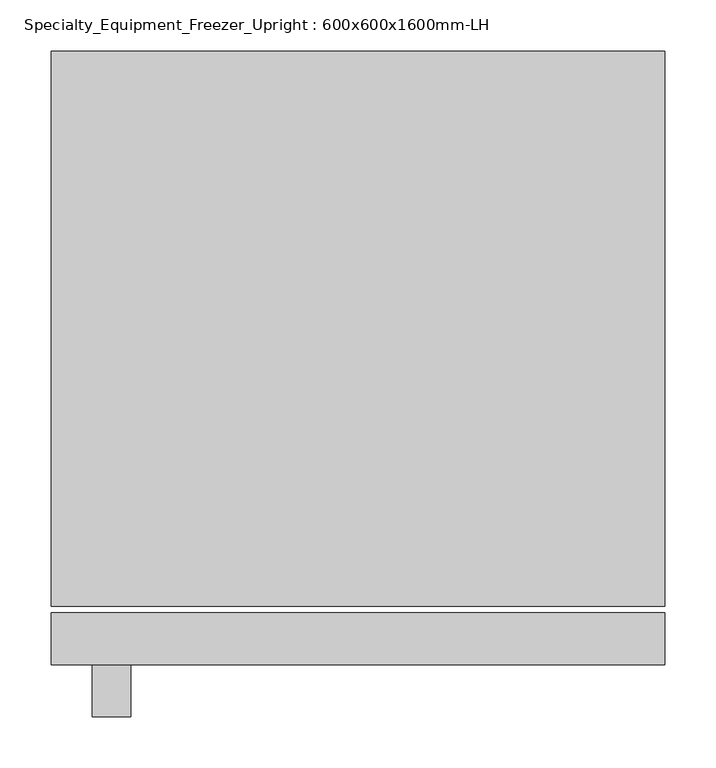
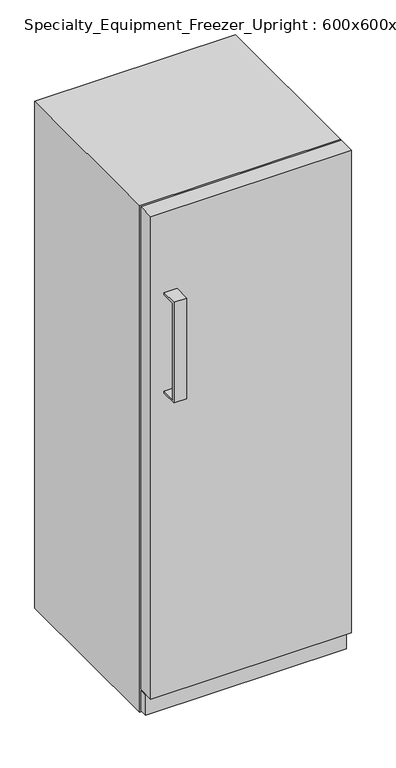
"""IFC4 building model written with IfcOpenShell, lengths in millimetres: proxy geometry, Specialty_Equipment_Freezer_Upright : 600x600x1600mm-LH."""

from ifc_helpers import new_model, si_unit, frame, origin, origin_with_axes, place, context, project, spatial, polyline, outline, extrude, source, transform, mapped, element, save


def specialty_equipment_freezer_upright_600x600x1600mm_lh_8c2ecadc(model_context):
    return source(origin(), model_context, "Body", "SweptSolid", [
        extrude(outline(polyline([(-314.6760285, 1339.65), (-359.1260285, 1339.65), (-359.1260285, 1034.85), (-314.6760285, 1034.85), (-314.6760285, 1028.5154683), (-365.4760285, 1028.5154683), (-365.4760285, 1346.0), (-314.6760285, 1346.0), (-314.6760285, 1339.65)])), frame((-260.0, 0.0, 0.0), z_axis=(1.0, 0.0, 0.0), x_axis=(0.0, 1.0, 0.0)), (0.0, 0.0, 1.0), 38.1),
        extrude(outline(polyline([(300.0, -263.8760285), (300.0, -289.2760285), (-300.0, -289.2760285), (-300.0, -263.8760285), (300.0, -263.8760285)])), frame((0.0, 0.0, 9.3816357), z_axis=(0.0, 0.0, 1.0), x_axis=(1.0, 0.0, 0.0)), (0.0, 0.0, 1.0), 63.5),
        extrude(outline(polyline([(300.0, -263.8760285), (300.0, -314.6760285), (-300.0, -314.6760285), (-300.0, -263.8760285), (300.0, -263.8760285)])), frame((0.0, 0.0, 76.2), z_axis=(0.0, 0.0, 1.0), x_axis=(1.0, 0.0, 0.0)), (0.0, 0.0, 1.0), 1523.8),
        extrude(outline(polyline([(300.0, 285.3239715), (300.0, -257.5260285), (-300.0, -257.5260285), (-300.0, 285.3239715), (300.0, 285.3239715)])), origin_with_axes(), (0.0, 0.0, 1.0), 1600.0),
    ])


if __name__ == "__main__":
    model = new_model("IFC4")
    model_context = context("Model", 3, world=origin())
    ifc_project = project(units=[si_unit("LENGTHUNIT", "METRE", prefix="MILLI")], contexts=[model_context])
    site = spatial("IfcSite", under=ifc_project)
    building = spatial("IfcBuilding", under=site)
    placement = place(None, origin())
    specialty_equipment_freezer_upright_600x600x1600mm_lh_shape = specialty_equipment_freezer_upright_600x600x1600mm_lh_8c2ecadc(model_context)
    element("IfcBuildingElementProxy", 1, Name="Specialty_Equipment_Freezer_Upright : 600x600x1600mm-LH", ObjectType="Specialty_Equipment_Freezer_Upright : 600x600x1600mm-LH", at=placement, inside=building, context=model_context, shape_type="MappedRepresentation", body=[
        mapped(specialty_equipment_freezer_upright_600x600x1600mm_lh_shape, transform((0.0, 0.0, 0.0), x_axis=(1.0, 0.0, 0.0), y_axis=(0.0, 1.0, 0.0), z_axis=(0.0, 0.0, 1.0))),
    ])
    save(model, "model.ifc")

# Revit data of these elements
# Type "Specialty_Equipment_Freezer_Upright : 600x600x1600mm-LH"
#   Type IfcGUID = "1aRjrFHzDDvwx1NU_3WgZx"
#   Classification.Uniclass.EF.Number = "EF_40_40"
#   Classification.Uniclass.EF.Description = "Equipment"
#   Keynote = "N10"
#   Assembly Code = "E1090400"
#   Depth = 0.6 m
#   Handle = 0.04 m
#   Height = 1.6 m
#   Rear Clearance = 0.05 m
#   Width = 0.6 m
#   Material = Metal - Paint Finish - Ivory, Glossy
#   Default Elevation = 0
# Element 1 (IfcBuildingElementProxy, "Specialty_Equipment_Freezer_Upright : 600x600x1600mm-LH")
#   Materials on its faces: "Metal - Paint Finish - Ivory, Glossy", "Metal - Chrome", "Metal - Paint Finish - Black, Glossy"
# Materials
#   "Metal - Paint Finish - Ivory, Glossy": class "Paint", colour RGB 247 247 239, transparency 0
#   "Metal - Chrome": class "Metal", colour RGB 247 247 247, transparency 0
#   "Metal - Paint Finish - Black, Glossy": class "Metal", colour RGB 0 0 0, transparency 0
